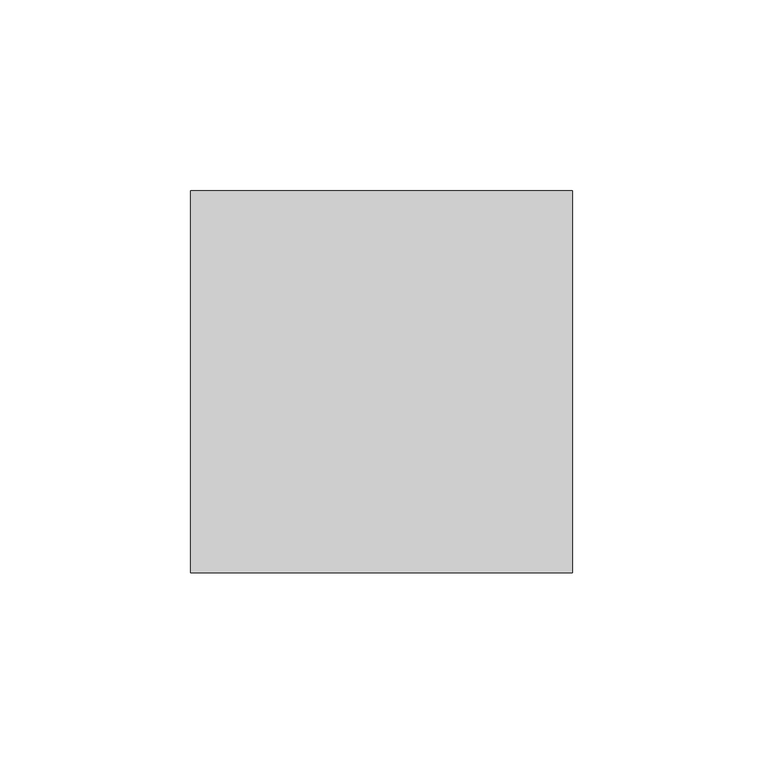
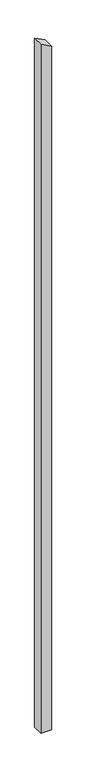
"""IFC4 building model written with IfcOpenShell, lengths in millimetres: column geometry, Holzstütze 159206 : Holzstütze 159206."""

import ifcopenshell
import ifcopenshell.guid

model = None  # the IFC model being written
_history = None  # IfcOwnerHistory: only IFC2X3 demands one
_inside = {}  # id of a spatial element -> (the spatial element, [elements in it])
_under = {}  # id of a project, library or spatial element -> (it, [spatial elements below it])
_declared = {}  # id of a project -> (the project, [libraries it declares])
_typed = {}  # id of a type object -> (the type object, [elements of that type])
_made_of = {}  # id of a material, layer set ... -> (it, [elements and type objects made of it])


def new_model(schema):
    """Start an empty IFC model of exactly this schema.

    Asked for "IFC4X3", IfcOpenShell would pick the latest addendum, in which some entities
    have other attributes; the version numbers below select the first issue.
    IFC2X3 requires an IfcOwnerHistory on every rooted entity: one is made here for all.
    """
    global model, _history
    if schema == "IFC4X3":
        model = ifcopenshell.file(schema_version=(4, 3, 0, 0))
    else:
        model = ifcopenshell.file(schema=schema)
    _inside.clear()
    _under.clear()
    _declared.clear()
    _typed.clear()
    _made_of.clear()
    _history = None
    if model.schema == "IFC2X3":
        org = make("IfcOrganization", Name="unknown")
        user = make(
            "IfcPersonAndOrganization",
            ThePerson=make("IfcPerson", FamilyName="unknown"),
            TheOrganization=org,
        )
        app = make(
            "IfcApplication",
            ApplicationDeveloper=org,
            Version="unknown",
            ApplicationFullName="unknown",
            ApplicationIdentifier="unknown",
        )
        _history = make(
            "IfcOwnerHistory",
            OwningUser=user,
            OwningApplication=app,
            ChangeAction="ADDED",
            CreationDate=0,
        )
    return model


def make(cls, **values):
    """One entity of the class cls with the attributes given. An attribute that is None is left unset."""
    return model.create_entity(
        cls, **{name: value for name, value in values.items() if value is not None}
    )


def rooted(cls, **values):
    """An entity with a GlobalId (a new one), such as an element, a storey or a relation."""
    return make(cls, GlobalId=ifcopenshell.guid.new(), OwnerHistory=_history, **values)


def si_unit(unit_type, name, prefix=None):
    """IfcSIUnit, for example si_unit("LENGTHUNIT", "METRE", prefix="MILLI")."""
    return make("IfcSIUnit", UnitType=unit_type, Prefix=prefix, Name=name)


def assignment(units):
    """IfcUnitAssignment: the units of a project."""
    return None if units is None else make("IfcUnitAssignment", Units=units)


def point(xyz):
    """IfcCartesianPoint."""
    return None if xyz is None else make("IfcCartesianPoint", Coordinates=xyz)


def direction(xyz):
    """IfcDirection."""
    return None if xyz is None else make("IfcDirection", DirectionRatios=xyz)


def frame(location, z_axis=None, x_axis=None):
    """IfcAxis2Placement3D, a coordinate frame: its origin and axes. An axis left out is left unset."""
    return make(
        "IfcAxis2Placement3D",
        Location=point(location),
        Axis=direction(z_axis),
        RefDirection=direction(x_axis),
    )


def origin():
    """The frame at (0, 0, 0) with its axes left unset."""
    return frame((0.0, 0.0, 0.0))


def place(relative_to, where):
    """IfcLocalPlacement: puts the frame where relative to a parent placement (None: the world)."""
    return make(
        "IfcLocalPlacement", PlacementRelTo=relative_to, RelativePlacement=where
    )


def context(
    kind, dimensions, precision=None, world=None, true_north=None, identifier=None
):
    """IfcGeometricRepresentationContext, for example the 3D "Model" context."""
    return make(
        "IfcGeometricRepresentationContext",
        ContextIdentifier=identifier,
        ContextType=kind,
        CoordinateSpaceDimension=dimensions,
        Precision=precision,
        WorldCoordinateSystem=world,
        TrueNorth=true_north,
    )


def project(units=None, contexts=None):
    """IfcProject with its units and contexts."""
    return rooted(
        "IfcProject",
        Name="project",
        RepresentationContexts=contexts,
        UnitsInContext=assignment(units),
    )


def spatial(cls, under=None, at=None, **own):
    """A site, building, storey or space (cls), placed at a placement, below another one or the project."""
    s = rooted(cls, ObjectPlacement=at, **own)
    if under is not None:
        _under.setdefault(under.id(), (under, []))[1].append(s)
    return s


def polyline(points):
    """IfcPolyline through the points."""
    return make("IfcPolyline", Points=[point(p) for p in points])


def outline(outer, holes=None, kind="AREA"):
    """IfcArbitraryClosedProfileDef: a profile drawn as a closed curve; with holes, ...WithVoids."""
    if holes is None:
        return make("IfcArbitraryClosedProfileDef", ProfileType=kind, OuterCurve=outer)
    return make(
        "IfcArbitraryProfileDefWithVoids",
        ProfileType=kind,
        OuterCurve=outer,
        InnerCurves=holes,
    )


def extrude(swept, where, along, depth):
    """IfcExtrudedAreaSolid: the profile swept, set in the frame where, extruded along a direction by depth."""
    return make(
        "IfcExtrudedAreaSolid",
        SweptArea=swept,
        Position=where,
        ExtrudedDirection=direction(along),
        Depth=depth,
    )


def shape(context_of_items, identifier, shape_type, items):
    """IfcShapeRepresentation: the items that make up one representation, for example the "Body"."""
    return make(
        "IfcShapeRepresentation",
        ContextOfItems=context_of_items,
        RepresentationIdentifier=identifier,
        RepresentationType=shape_type,
        Items=items,
    )


def source(mapping_origin, context_of_items, identifier, shape_type, items):
    """IfcRepresentationMap: a shape defined once, which mapped items show again and again."""
    return make(
        "IfcRepresentationMap",
        MappingOrigin=mapping_origin,
        MappedRepresentation=shape(context_of_items, identifier, shape_type, items),
    )


def transform(
    local_origin,
    x_axis=None,
    y_axis=None,
    z_axis=None,
    scale=None,
    scale2=None,
    scale3=None,
    uniform=True,
):
    """IfcCartesianTransformationOperator3D, or its non-uniform kind. x_axis, y_axis, z_axis: its Axis1, 2, 3."""
    if uniform:
        return make(
            "IfcCartesianTransformationOperator3D",
            Axis1=direction(x_axis),
            Axis2=direction(y_axis),
            LocalOrigin=point(local_origin),
            Scale=scale,
            Axis3=direction(z_axis),
        )
    return make(
        "IfcCartesianTransformationOperator3DnonUniform",
        Axis1=direction(x_axis),
        Axis2=direction(y_axis),
        LocalOrigin=point(local_origin),
        Scale=scale,
        Axis3=direction(z_axis),
        Scale2=scale2,
        Scale3=scale3,
    )


def mapped(mapping_source, mapping_target):
    """IfcMappedItem: shows the shape of a source again, moved by a transform."""
    return make(
        "IfcMappedItem", MappingSource=mapping_source, MappingTarget=mapping_target
    )


def made_of(thing, what):
    """Note that an element or type object is made of a material, layer set ...; save() writes the relation."""
    if what is not None:
        _made_of.setdefault(what.id(), (what, []))[1].append(thing)
    return thing


def element(
    cls,
    number,
    at=None,
    inside=None,
    cuts=None,
    type_object=None,
    material=None,
    context=None,
    identifier="Body",
    shape_type=None,
    held_by="IfcProductDefinitionShape",
    body=None,
    shapes=None,
    **own,
):
    """One element of the class cls, such as IfcWall. Its Tag is "e" and its number.

    at: its placement. inside: the storey or other place that contains it. cuts: it is an
    opening in that element (IfcRelVoidsElement). A single representation is given by context,
    identifier, shape_type and body (its items); several are given by shapes. held_by: the class
    of the entity that holds the representations. save() writes the other relations.
    """
    e = rooted(cls, Tag="e%d" % number, ObjectPlacement=at, **own)
    if body is not None:
        shapes = [shape(context, identifier, shape_type, body)]
    if shapes is not None:
        e.Representation = make(held_by, Representations=shapes)
    if inside is not None:
        _inside.setdefault(inside.id(), (inside, []))[1].append(e)
    if cuts is not None:
        rooted(
            "IfcRelVoidsElement", RelatingBuildingElement=cuts, RelatedOpeningElement=e
        )
    if type_object is not None:
        _typed.setdefault(type_object.id(), (type_object, []))[1].append(e)
    return made_of(e, material)


def aggregate(whole, parts):
    """IfcRelAggregates: a whole, such as a stair, and the parts it consists of."""
    return rooted("IfcRelAggregates", RelatingObject=whole, RelatedObjects=parts)


def save(model, path):
    """Write the relations noted so far, then the file.

    IfcRelAggregates (storeys below a building ...), IfcRelContainedInSpatialStructure (elements
    in a storey), IfcRelDefinesByType, IfcRelAssociatesMaterial and IfcRelDeclares: one each for
    every whole, place, type object, material and project.
    """
    for whole, parts in _under.values():
        aggregate(whole, parts)
    for where, things in _inside.values():
        rooted(
            "IfcRelContainedInSpatialStructure",
            RelatedElements=things,
            RelatingStructure=where,
        )
    for kind, things in _typed.values():
        rooted("IfcRelDefinesByType", RelatedObjects=things, RelatingType=kind)
    for what, things in _made_of.values():
        rooted("IfcRelAssociatesMaterial", RelatedObjects=things, RelatingMaterial=what)
    for by, libraries in _declared.values():
        rooted("IfcRelDeclares", RelatingContext=by, RelatedDefinitions=libraries)
    model.write(path)


def column_acd7d749(model_context):
    return source(origin(), model_context, "Body", "SweptSolid", [
        extrude(outline(polyline([(-500.0, 174197.7593015), (-500.0, 174297.7593015), (6345.7118258, 174297.7593015), (6396.6643707, 174197.7593015), (-500.0, 174197.7593015)])), frame((0.0, 35528.3551606, 0.0), z_axis=(0.0, 1.0, 0.0), x_axis=(0.0, 0.0, 1.0)), (0.0, 0.0, 1.0), 100.0),
    ])


if __name__ == "__main__":
    model = new_model("IFC4")
    model_context = context("Model", 3, world=origin())
    ifc_project = project(units=[si_unit("LENGTHUNIT", "METRE", prefix="MILLI")], contexts=[model_context])
    site = spatial("IfcSite", under=ifc_project)
    building = spatial("IfcBuilding", under=site)
    placement = place(None, origin())
    column_shape = column_acd7d749(model_context)
    element("IfcColumn", 1, ObjectType="Holzstütze 159206 : Holzstütze 159206", at=placement, inside=building, context=model_context, shape_type="MappedRepresentation", body=[
        mapped(column_shape, transform((0.0, 0.0, 0.0), x_axis=(1.0, 0.0, 0.0), y_axis=(0.0, 1.0, 0.0), z_axis=(0.0, 0.0, 1.0))),
    ])
    save(model, "model.ifc")

# Revit data of these elements
# Type "Holzstütze 159206 : Holzstütze 159206"
#   Abrechnungsart = "m"
#   Allright_Bauteil_ID = "0152St 0000143482"
#   Bezeichnung = "Holzstütze"
#   Codetext = "ST-HOLZ\\"
#   Gewerk = "Zimmer- und Holzbauarbeiten"
#   Material = "Holz"
#   Objektname = "Stütze"
#   NameOverride = "Holzstütze"
#   Reference = "Holzstütze"
#   Status = "NEW"
#   ThermalTransmittance = 0.0000 BTU/(h·ft²·°F)
#   Roll = 0.00°
#   Slope = 0.00°
#   2D Interaktion = yes
#   IsExternal = yes
#   LoadBearing = yes
# Element 1 (IfcColumn, "Holzstütze 159206 : Holzstütze 159206")
#   Materials on its faces: "holzschalung"
# Materials
#   "holzschalung": class "Unassigned", colour RGB 128 128 128, transparency 0
